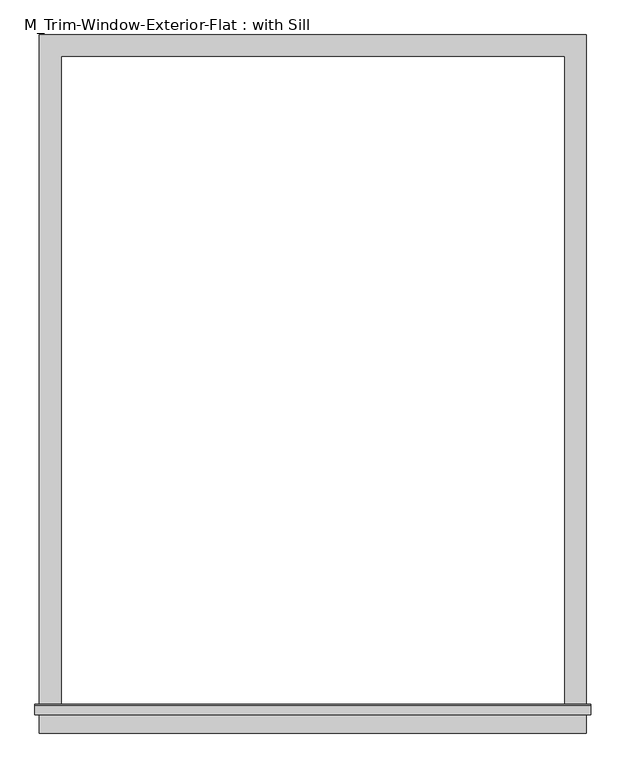
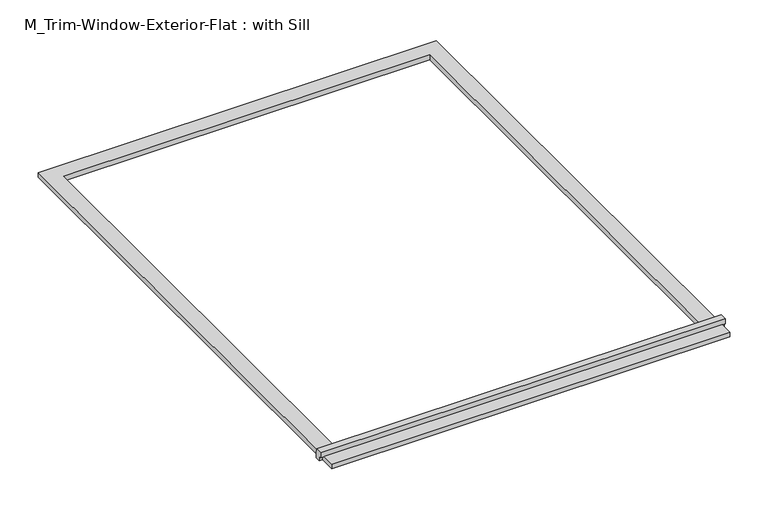
"""IFC4 building model written with IfcOpenShell, lengths in millimetres: proxy geometry, M_Trim-Window-Exterior-Flat : with Sill."""

import ifcopenshell
import ifcopenshell.guid

model = None  # the IFC model being written
_history = None  # IfcOwnerHistory: only IFC2X3 demands one
_inside = {}  # id of a spatial element -> (the spatial element, [elements in it])
_under = {}  # id of a project, library or spatial element -> (it, [spatial elements below it])
_declared = {}  # id of a project -> (the project, [libraries it declares])
_typed = {}  # id of a type object -> (the type object, [elements of that type])
_made_of = {}  # id of a material, layer set ... -> (it, [elements and type objects made of it])


def new_model(schema):
    """Start an empty IFC model of exactly this schema.

    Asked for "IFC4X3", IfcOpenShell would pick the latest addendum, in which some entities
    have other attributes; the version numbers below select the first issue.
    IFC2X3 requires an IfcOwnerHistory on every rooted entity: one is made here for all.
    """
    global model, _history
    if schema == "IFC4X3":
        model = ifcopenshell.file(schema_version=(4, 3, 0, 0))
    else:
        model = ifcopenshell.file(schema=schema)
    _inside.clear()
    _under.clear()
    _declared.clear()
    _typed.clear()
    _made_of.clear()
    _history = None
    if model.schema == "IFC2X3":
        org = make("IfcOrganization", Name="unknown")
        user = make(
            "IfcPersonAndOrganization",
            ThePerson=make("IfcPerson", FamilyName="unknown"),
            TheOrganization=org,
        )
        app = make(
            "IfcApplication",
            ApplicationDeveloper=org,
            Version="unknown",
            ApplicationFullName="unknown",
            ApplicationIdentifier="unknown",
        )
        _history = make(
            "IfcOwnerHistory",
            OwningUser=user,
            OwningApplication=app,
            ChangeAction="ADDED",
            CreationDate=0,
        )
    return model


def make(cls, **values):
    """One entity of the class cls with the attributes given. An attribute that is None is left unset."""
    return model.create_entity(
        cls, **{name: value for name, value in values.items() if value is not None}
    )


def rooted(cls, **values):
    """An entity with a GlobalId (a new one), such as an element, a storey or a relation."""
    return make(cls, GlobalId=ifcopenshell.guid.new(), OwnerHistory=_history, **values)


def si_unit(unit_type, name, prefix=None):
    """IfcSIUnit, for example si_unit("LENGTHUNIT", "METRE", prefix="MILLI")."""
    return make("IfcSIUnit", UnitType=unit_type, Prefix=prefix, Name=name)


def assignment(units):
    """IfcUnitAssignment: the units of a project."""
    return None if units is None else make("IfcUnitAssignment", Units=units)


def point(xyz):
    """IfcCartesianPoint."""
    return None if xyz is None else make("IfcCartesianPoint", Coordinates=xyz)


def direction(xyz):
    """IfcDirection."""
    return None if xyz is None else make("IfcDirection", DirectionRatios=xyz)


def frame(location, z_axis=None, x_axis=None):
    """IfcAxis2Placement3D, a coordinate frame: its origin and axes. An axis left out is left unset."""
    return make(
        "IfcAxis2Placement3D",
        Location=point(location),
        Axis=direction(z_axis),
        RefDirection=direction(x_axis),
    )


def origin():
    """The frame at (0, 0, 0) with its axes left unset."""
    return frame((0.0, 0.0, 0.0))


def origin_with_axes():
    """The frame at (0, 0, 0) with the z axis (0, 0, 1) and the x axis (1, 0, 0) written out."""
    return frame((0.0, 0.0, 0.0), z_axis=(0.0, 0.0, 1.0), x_axis=(1.0, 0.0, 0.0))


def place(relative_to, where):
    """IfcLocalPlacement: puts the frame where relative to a parent placement (None: the world)."""
    return make(
        "IfcLocalPlacement", PlacementRelTo=relative_to, RelativePlacement=where
    )


def context(
    kind, dimensions, precision=None, world=None, true_north=None, identifier=None
):
    """IfcGeometricRepresentationContext, for example the 3D "Model" context."""
    return make(
        "IfcGeometricRepresentationContext",
        ContextIdentifier=identifier,
        ContextType=kind,
        CoordinateSpaceDimension=dimensions,
        Precision=precision,
        WorldCoordinateSystem=world,
        TrueNorth=true_north,
    )


def project(units=None, contexts=None):
    """IfcProject with its units and contexts."""
    return rooted(
        "IfcProject",
        Name="project",
        RepresentationContexts=contexts,
        UnitsInContext=assignment(units),
    )


def spatial(cls, under=None, at=None, **own):
    """A site, building, storey or space (cls), placed at a placement, below another one or the project."""
    s = rooted(cls, ObjectPlacement=at, **own)
    if under is not None:
        _under.setdefault(under.id(), (under, []))[1].append(s)
    return s


def polyline(points):
    """IfcPolyline through the points."""
    return make("IfcPolyline", Points=[point(p) for p in points])


def outline(outer, holes=None, kind="AREA"):
    """IfcArbitraryClosedProfileDef: a profile drawn as a closed curve; with holes, ...WithVoids."""
    if holes is None:
        return make("IfcArbitraryClosedProfileDef", ProfileType=kind, OuterCurve=outer)
    return make(
        "IfcArbitraryProfileDefWithVoids",
        ProfileType=kind,
        OuterCurve=outer,
        InnerCurves=holes,
    )


def extrude(swept, where, along, depth):
    """IfcExtrudedAreaSolid: the profile swept, set in the frame where, extruded along a direction by depth."""
    return make(
        "IfcExtrudedAreaSolid",
        SweptArea=swept,
        Position=where,
        ExtrudedDirection=direction(along),
        Depth=depth,
    )


def shape(context_of_items, identifier, shape_type, items):
    """IfcShapeRepresentation: the items that make up one representation, for example the "Body"."""
    return make(
        "IfcShapeRepresentation",
        ContextOfItems=context_of_items,
        RepresentationIdentifier=identifier,
        RepresentationType=shape_type,
        Items=items,
    )


def source(mapping_origin, context_of_items, identifier, shape_type, items):
    """IfcRepresentationMap: a shape defined once, which mapped items show again and again."""
    return make(
        "IfcRepresentationMap",
        MappingOrigin=mapping_origin,
        MappedRepresentation=shape(context_of_items, identifier, shape_type, items),
    )


def transform(
    local_origin,
    x_axis=None,
    y_axis=None,
    z_axis=None,
    scale=None,
    scale2=None,
    scale3=None,
    uniform=True,
):
    """IfcCartesianTransformationOperator3D, or its non-uniform kind. x_axis, y_axis, z_axis: its Axis1, 2, 3."""
    if uniform:
        return make(
            "IfcCartesianTransformationOperator3D",
            Axis1=direction(x_axis),
            Axis2=direction(y_axis),
            LocalOrigin=point(local_origin),
            Scale=scale,
            Axis3=direction(z_axis),
        )
    return make(
        "IfcCartesianTransformationOperator3DnonUniform",
        Axis1=direction(x_axis),
        Axis2=direction(y_axis),
        LocalOrigin=point(local_origin),
        Scale=scale,
        Axis3=direction(z_axis),
        Scale2=scale2,
        Scale3=scale3,
    )


def mapped(mapping_source, mapping_target):
    """IfcMappedItem: shows the shape of a source again, moved by a transform."""
    return make(
        "IfcMappedItem", MappingSource=mapping_source, MappingTarget=mapping_target
    )


def made_of(thing, what):
    """Note that an element or type object is made of a material, layer set ...; save() writes the relation."""
    if what is not None:
        _made_of.setdefault(what.id(), (what, []))[1].append(thing)
    return thing


def element(
    cls,
    number,
    at=None,
    inside=None,
    cuts=None,
    type_object=None,
    material=None,
    context=None,
    identifier="Body",
    shape_type=None,
    held_by="IfcProductDefinitionShape",
    body=None,
    shapes=None,
    **own,
):
    """One element of the class cls, such as IfcWall. Its Tag is "e" and its number.

    at: its placement. inside: the storey or other place that contains it. cuts: it is an
    opening in that element (IfcRelVoidsElement). A single representation is given by context,
    identifier, shape_type and body (its items); several are given by shapes. held_by: the class
    of the entity that holds the representations. save() writes the other relations.
    """
    e = rooted(cls, Tag="e%d" % number, ObjectPlacement=at, **own)
    if body is not None:
        shapes = [shape(context, identifier, shape_type, body)]
    if shapes is not None:
        e.Representation = make(held_by, Representations=shapes)
    if inside is not None:
        _inside.setdefault(inside.id(), (inside, []))[1].append(e)
    if cuts is not None:
        rooted(
            "IfcRelVoidsElement", RelatingBuildingElement=cuts, RelatedOpeningElement=e
        )
    if type_object is not None:
        _typed.setdefault(type_object.id(), (type_object, []))[1].append(e)
    return made_of(e, material)


def aggregate(whole, parts):
    """IfcRelAggregates: a whole, such as a stair, and the parts it consists of."""
    return rooted("IfcRelAggregates", RelatingObject=whole, RelatedObjects=parts)


def save(model, path):
    """Write the relations noted so far, then the file.

    IfcRelAggregates (storeys below a building ...), IfcRelContainedInSpatialStructure (elements
    in a storey), IfcRelDefinesByType, IfcRelAssociatesMaterial and IfcRelDeclares: one each for
    every whole, place, type object, material and project.
    """
    for whole, parts in _under.values():
        aggregate(whole, parts)
    for where, things in _inside.values():
        rooted(
            "IfcRelContainedInSpatialStructure",
            RelatedElements=things,
            RelatingStructure=where,
        )
    for kind, things in _typed.values():
        rooted("IfcRelDefinesByType", RelatedObjects=things, RelatingType=kind)
    for what, things in _made_of.values():
        rooted("IfcRelAssociatesMaterial", RelatedObjects=things, RelatingMaterial=what)
    for by, libraries in _declared.values():
        rooted("IfcRelDeclares", RelatingContext=by, RelatedDefinitions=libraries)
    model.write(path)


def m_trim_window_exterior_flat_with_sill_136e302d(model_context):
    return source(origin(), model_context, "Body", "SweptSolid", [
        extrude(outline(polyline([(760.0, -1820.4323709), (760.0, -1880.4323709), (-760.0, -1880.4323709), (-760.0, -1820.4323709), (760.0, -1820.4323709)])), origin_with_axes(), (0.0, 0.0, 1.0), 19.05),
        extrude(outline(polyline([(-1830.0, 38.1), (-1802.4580645, 38.1), (-1800.0, 19.05), (-1800.0, 0.0), (-1820.4323709, 0.0), (-1820.4323709, 19.05), (-1830.0, 19.05), (-1830.0, 38.1)])), frame((-772.7, 0.0, 0.0), z_axis=(1.0, 0.0, 0.0), x_axis=(0.0, 1.0, 0.0)), (0.0, 0.0, 1.0), 1545.4),
        extrude(outline(polyline([(-760.0, 60.0), (760.0, 60.0), (760.0, -1800.0), (700.0, -1800.0), (700.0, 0.0), (-700.0, 0.0), (-700.0, -1800.0), (-760.0, -1800.0), (-760.0, 60.0)])), origin_with_axes(), (0.0, 0.0, 1.0), 19.05),
    ])


if __name__ == "__main__":
    model = new_model("IFC4")
    model_context = context("Model", 3, world=origin())
    ifc_project = project(units=[si_unit("LENGTHUNIT", "METRE", prefix="MILLI")], contexts=[model_context])
    site = spatial("IfcSite", under=ifc_project)
    building = spatial("IfcBuilding", under=site)
    placement = place(None, origin())
    m_trim_window_exterior_flat_with_sill_shape = m_trim_window_exterior_flat_with_sill_136e302d(model_context)
    element("IfcBuildingElementProxy", 1, Name="M_Trim-Window-Exterior-Flat : with Sill", ObjectType="M_Trim-Window-Exterior-Flat : with Sill", at=placement, inside=building, context=model_context, shape_type="MappedRepresentation", body=[
        mapped(m_trim_window_exterior_flat_with_sill_shape, transform((0.0, 0.0, 0.0), x_axis=(1.0, 0.0, 0.0), y_axis=(0.0, 1.0, 0.0), z_axis=(0.0, 0.0, 1.0))),
    ])
    save(model, "model.ifc")

# Revit data of these elements
# Type "M_Trim-Window-Exterior-Flat : with Sill"
#   Trim Width = 6 cm
#   Trim Thickness_Picture Frame = 3 cm
#   Trim Thickness_with Sill = 1.905 cm
#   Sill Thickness = 3 cm
#   Opening Width [instance default] = 60 cm
#   Opening Height [instance default] = 90 cm
#   Default Elevation = 120 cm
#   Sill = yes
#   Picture Frame = no
#   Trim Material [instance default] = none
# Element 1 (IfcBuildingElementProxy, "M_Trim-Window-Exterior-Flat : with Sill")
#   Opening Width = 140 cm
#   Opening Height = 180 cm
#   Trim Material = Clad - White
#   Materials on its faces: "Clad - White"
# Materials
#   "Clad - White": class "Wood", colour RGB 242 242 238, transparency 0, Cost = 0
